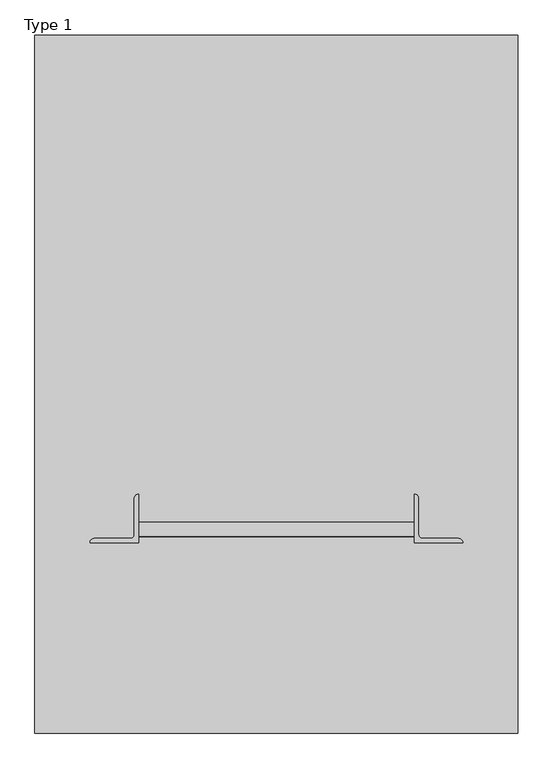
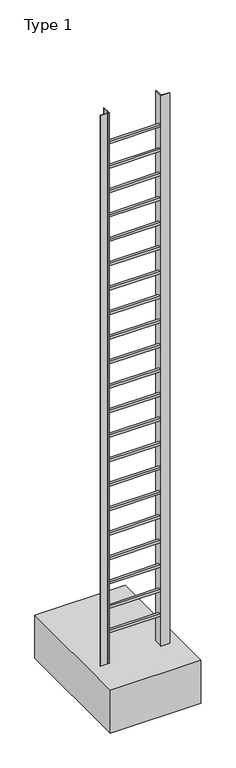
"""IFC4 building model written with IfcOpenShell, lengths in millimetres: proxy geometry, LF03GAK001_LADDER_NML_rAD : Type 1."""

from ifc_helpers import new_model, si_unit, point, frame, frame_2d, origin, place, context, project, spatial, polyline, circle_curve, trimmed, segment, composite_curve, outline, extrude, source, transform, mapped, element, save


def type_1_dbdeaf5a(model_context):
    return source(origin(), model_context, "Body", "SweptSolid", [
        extrude(outline(polyline([(325.0, 379.3), (325.0, 359.3), (-75.0, 359.3), (-75.0, 379.3), (325.0, 379.3)])), frame((0.0, 0.0, 4390.0), z_axis=(0.0, 0.0, 1.0), x_axis=(1.0, 0.0, 0.0)), (0.0, 0.0, 1.0), 20.0),
        extrude(outline(polyline([(325.0, 379.3), (325.0, 359.3), (-75.0, 359.3), (-75.0, 379.3), (325.0, 379.3)])), frame((0.0, 0.0, 4190.0), z_axis=(0.0, 0.0, 1.0), x_axis=(1.0, 0.0, 0.0)), (0.0, 0.0, 1.0), 20.0),
        extrude(outline(polyline([(325.0, 379.3), (325.0, 359.3), (-75.0, 359.3), (-75.0, 379.3), (325.0, 379.3)])), frame((0.0, 0.0, 3990.0), z_axis=(0.0, 0.0, 1.0), x_axis=(1.0, 0.0, 0.0)), (0.0, 0.0, 1.0), 20.0),
        extrude(outline(polyline([(325.0, 379.3), (325.0, 359.3), (-75.0, 359.3), (-75.0, 379.3), (325.0, 379.3)])), frame((0.0, 0.0, 3790.0), z_axis=(0.0, 0.0, 1.0), x_axis=(1.0, 0.0, 0.0)), (0.0, 0.0, 1.0), 20.0),
        extrude(outline(polyline([(325.0, 379.3), (325.0, 359.3), (-75.0, 359.3), (-75.0, 379.3), (325.0, 379.3)])), frame((0.0, 0.0, 3590.0), z_axis=(0.0, 0.0, 1.0), x_axis=(1.0, 0.0, 0.0)), (0.0, 0.0, 1.0), 20.0),
        extrude(outline(polyline([(325.0, 379.3), (325.0, 359.3), (-75.0, 359.3), (-75.0, 379.3), (325.0, 379.3)])), frame((0.0, 0.0, 3390.0), z_axis=(0.0, 0.0, 1.0), x_axis=(1.0, 0.0, 0.0)), (0.0, 0.0, 1.0), 20.0),
        extrude(outline(polyline([(325.0, 379.3), (325.0, 359.3), (-75.0, 359.3), (-75.0, 379.3), (325.0, 379.3)])), frame((0.0, 0.0, 3190.0), z_axis=(0.0, 0.0, 1.0), x_axis=(1.0, 0.0, 0.0)), (0.0, 0.0, 1.0), 20.0),
        extrude(outline(polyline([(325.0, 379.3), (325.0, 359.3), (-75.0, 359.3), (-75.0, 379.3), (325.0, 379.3)])), frame((0.0, 0.0, 2990.0), z_axis=(0.0, 0.0, 1.0), x_axis=(1.0, 0.0, 0.0)), (0.0, 0.0, 1.0), 20.0),
        extrude(outline(polyline([(325.0, 379.3), (325.0, 359.3), (-75.0, 359.3), (-75.0, 379.3), (325.0, 379.3)])), frame((0.0, 0.0, 2790.0), z_axis=(0.0, 0.0, 1.0), x_axis=(1.0, 0.0, 0.0)), (0.0, 0.0, 1.0), 20.0),
        extrude(outline(polyline([(325.0, 379.3), (325.0, 359.3), (-75.0, 359.3), (-75.0, 379.3), (325.0, 379.3)])), frame((0.0, 0.0, 2590.0), z_axis=(0.0, 0.0, 1.0), x_axis=(1.0, 0.0, 0.0)), (0.0, 0.0, 1.0), 20.0),
        extrude(outline(polyline([(325.0, 379.3), (325.0, 359.3), (-75.0, 359.3), (-75.0, 379.3), (325.0, 379.3)])), frame((0.0, 0.0, 2390.0), z_axis=(0.0, 0.0, 1.0), x_axis=(1.0, 0.0, 0.0)), (0.0, 0.0, 1.0), 20.0),
        extrude(outline(composite_curve([segment(polyline([(-75.0, 350.0), (-145.0, 350.0)]), True, "CONTINUOUS"), segment(trimmed(circle_curve(frame_2d((-139.0, 350.0)), 6.0), [point((-145.0, 350.0))], [point((-139.0, 356.0))], False, "CARTESIAN"), True, "CONTINUOUS"), segment(polyline([(-139.0, 356.0), (-87.0, 356.0)]), True, "CONTINUOUS"), segment(trimmed(circle_curve(frame_2d((-87.0, 362.0)), 6.0), [point((-87.0, 356.0))], [point((-81.0, 362.0))], True, "CARTESIAN"), True, "CONTINUOUS"), segment(polyline([(-81.0, 362.0), (-81.0, 414.0)]), True, "CONTINUOUS"), segment(trimmed(circle_curve(frame_2d((-75.0, 414.0)), 6.0), [point((-81.0, 414.0))], [point((-75.0, 420.0))], False, "CARTESIAN"), True, "CONTINUOUS"), segment(polyline([(-75.0, 420.0), (-75.0, 350.0)]), True, "CONTINUOUS")], self_intersect=False)), frame((0.0, 0.0, 150.0), z_axis=(0.0, 0.0, 1.0), x_axis=(1.0, 0.0, 0.0)), (0.0, 0.0, 1.0), 4500.0),
        extrude(outline(polyline([(325.0, 379.3), (325.0, 359.3), (-75.0, 359.3), (-75.0, 379.3), (325.0, 379.3)])), frame((0.0, 0.0, 2190.0), z_axis=(0.0, 0.0, 1.0), x_axis=(1.0, 0.0, 0.0)), (0.0, 0.0, 1.0), 20.0),
        extrude(outline(polyline([(325.0, 379.3), (325.0, 359.3), (-75.0, 359.3), (-75.0, 379.3), (325.0, 379.3)])), frame((0.0, 0.0, 1990.0), z_axis=(0.0, 0.0, 1.0), x_axis=(1.0, 0.0, 0.0)), (0.0, 0.0, 1.0), 20.0),
        extrude(outline(polyline([(325.0, 379.3), (325.0, 359.3), (-75.0, 359.3), (-75.0, 379.3), (325.0, 379.3)])), frame((0.0, 0.0, 1790.0), z_axis=(0.0, 0.0, 1.0), x_axis=(1.0, 0.0, 0.0)), (0.0, 0.0, 1.0), 20.0),
        extrude(outline(polyline([(325.0, 379.3), (325.0, 359.3), (-75.0, 359.3), (-75.0, 379.3), (325.0, 379.3)])), frame((0.0, 0.0, 1590.0), z_axis=(0.0, 0.0, 1.0), x_axis=(1.0, 0.0, 0.0)), (0.0, 0.0, 1.0), 20.0),
        extrude(outline(polyline([(325.0, 379.3), (325.0, 359.3), (-75.0, 359.3), (-75.0, 379.3), (325.0, 379.3)])), frame((0.0, 0.0, 1390.0), z_axis=(0.0, 0.0, 1.0), x_axis=(1.0, 0.0, 0.0)), (0.0, 0.0, 1.0), 20.0),
        extrude(outline(polyline([(325.0, 379.3), (325.0, 359.3), (-75.0, 359.3), (-75.0, 379.3), (325.0, 379.3)])), frame((0.0, 0.0, 1190.0), z_axis=(0.0, 0.0, 1.0), x_axis=(1.0, 0.0, 0.0)), (0.0, 0.0, 1.0), 20.0),
        extrude(outline(polyline([(325.0, 379.3), (325.0, 359.3), (-75.0, 359.3), (-75.0, 379.3), (325.0, 379.3)])), frame((0.0, 0.0, 990.0), z_axis=(0.0, 0.0, 1.0), x_axis=(1.0, 0.0, 0.0)), (0.0, 0.0, 1.0), 20.0),
        extrude(outline(polyline([(325.0, 379.3), (325.0, 359.3), (-75.0, 359.3), (-75.0, 379.3), (325.0, 379.3)])), frame((0.0, 0.0, 790.0), z_axis=(0.0, 0.0, 1.0), x_axis=(1.0, 0.0, 0.0)), (0.0, 0.0, 1.0), 20.0),
        extrude(outline(polyline([(325.0, 379.3), (325.0, 359.3), (-75.0, 359.3), (-75.0, 379.3), (325.0, 379.3)])), frame((0.0, 0.0, 590.0), z_axis=(0.0, 0.0, 1.0), x_axis=(1.0, 0.0, 0.0)), (0.0, 0.0, 1.0), 20.0),
        extrude(outline(polyline([(325.0, 379.3), (325.0, 359.3), (-75.0, 359.3), (-75.0, 379.3), (325.0, 379.3)])), frame((0.0, 0.0, 390.0), z_axis=(0.0, 0.0, 1.0), x_axis=(1.0, 0.0, 0.0)), (0.0, 0.0, 1.0), 20.0),
        extrude(outline(composite_curve([segment(polyline([(325.0, 350.0), (325.0, 420.0)]), True, "CONTINUOUS"), segment(trimmed(circle_curve(frame_2d((325.0, 414.0)), 6.0), [point((325.0, 420.0))], [point((331.0, 414.0))], False, "CARTESIAN"), True, "CONTINUOUS"), segment(polyline([(331.0, 414.0), (331.0, 362.0)]), True, "CONTINUOUS"), segment(trimmed(circle_curve(frame_2d((337.0, 362.0)), 6.0), [point((331.0, 362.0))], [point((337.0, 356.0))], True, "CARTESIAN"), True, "CONTINUOUS"), segment(polyline([(337.0, 356.0), (389.0, 356.0)]), True, "CONTINUOUS"), segment(trimmed(circle_curve(frame_2d((389.0, 350.0)), 6.0), [point((389.0, 356.0))], [point((395.0, 350.0))], False, "CARTESIAN"), True, "CONTINUOUS"), segment(polyline([(395.0, 350.0), (325.0, 350.0)]), True, "CONTINUOUS")], self_intersect=False)), frame((0.0, 0.0, 150.0), z_axis=(0.0, 0.0, 1.0), x_axis=(1.0, 0.0, 0.0)), (0.0, 0.0, 1.0), 4500.0),
        extrude(outline(polyline([(475.0, 1085.0), (475.0, 75.0), (-225.0, 75.0), (-225.0, 1085.0), (475.0, 1085.0)])), frame((0.0, 0.0, -200.0), z_axis=(0.0, 0.0, 1.0), x_axis=(1.0, 0.0, 0.0)), (0.0, 0.0, 1.0), 350.0),
    ])


if __name__ == "__main__":
    model = new_model("IFC4")
    model_context = context("Model", 3, world=origin())
    ifc_project = project(units=[si_unit("LENGTHUNIT", "METRE", prefix="MILLI")], contexts=[model_context])
    site = spatial("IfcSite", under=ifc_project)
    building = spatial("IfcBuilding", under=site)
    placement = place(None, origin())
    type_1_shape = type_1_dbdeaf5a(model_context)
    element("IfcBuildingElementProxy", 1, Name="LF03GAK001_LADDER_NML_rAD : Type 1", ObjectType="LF03GAK001_LADDER_NML_rAD : Type 1", at=placement, inside=building, context=model_context, shape_type="MappedRepresentation", body=[
        mapped(type_1_shape, transform((0.0, 0.0, 0.0), x_axis=(1.0, 0.0, 0.0), y_axis=(0.0, 1.0, 0.0), z_axis=(0.0, 0.0, 1.0))),
    ])
    save(model, "model.ifc")

# Revit data of these elements
# Type "LF03GAK001_LADDER_NML_rAD : Type 1"
#   ld_total height [instance default] = 2500 mm
#   ld_rung size [instance default] = 20 mm
#   ld_rung posi_hori = 19.3 mm
#   ld_rung dist_first [instance default] = 300 mm
#   ld_pad width [instance default] = 700 mm
#   ld_pad to mf center = 150 mm
#   ld_pad length [instance default] = 850 mm
#   ld_pad height [instance default] = 150 mm
#   ld_main distance [instance default] = 400 mm
#   ld_dist_to wall = 350 mm
#   ld_rung spacing [instance default] = 200 mm
#   ld_number of rungs [instance default] = 10
#   c1_material [instance default] = none
#   Default Elevation = 0
# Element 1 (IfcBuildingElementProxy, "LF03GAK001_LADDER_NML_rAD : Type 1")
#   ld_total height = 4650 mm
#   ld_rung dist_first = 250 mm
#   ld_number of rungs = 21
#   Materials on its faces: "금속 - 스틸 - 345MPa"
# Materials
#   "금속 - 스틸 - 345MPa": class "금속", colour RGB 247 247 247, transparency 0
